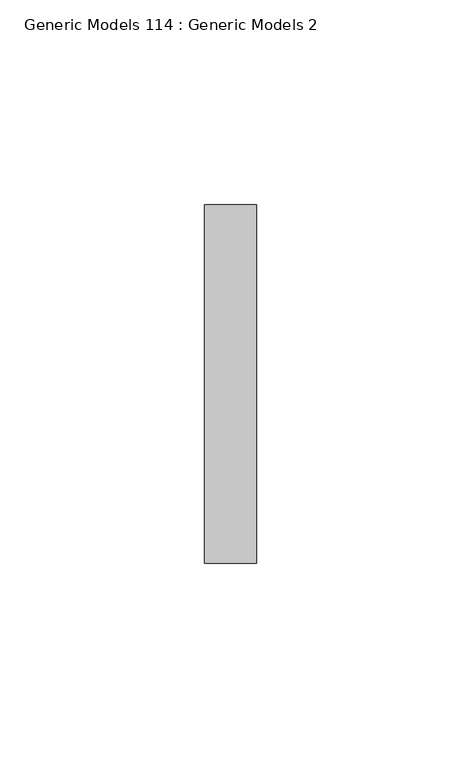
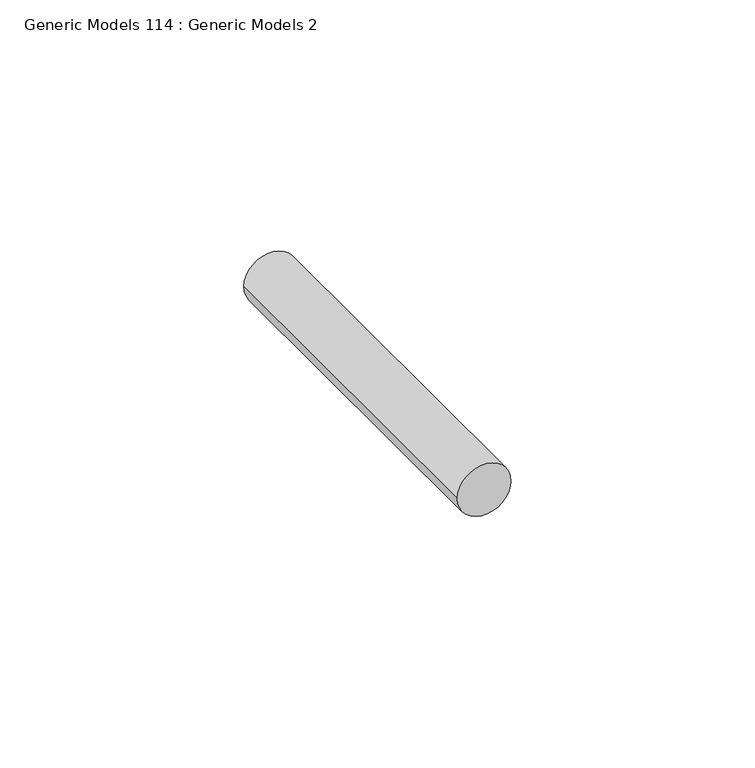
"""IFC4 building model written with IfcOpenShell, lengths in millimetres: proxy geometry, Generic Models 114 : Generic Models 2."""

from ifc_helpers import new_model, si_unit, point, frame, frame_2d, origin, place, context, project, spatial, circle_curve, trimmed, segment, composite_curve, outline, extrude, source, transform, mapped, element, save


def generic_models_114_generic_models_2_6e7f5802(model_context):
    return source(origin(), model_context, "Body", "SweptSolid", [
        extrude(outline(composite_curve([segment(trimmed(circle_curve(frame_2d((37860.4162436, 6848.7828124)), 6.35), [point((37860.4162436, 6842.4328124))], [point((37860.4162436, 6855.1328124))], False, "CARTESIAN"), True, "CONTINUOUS"), segment(trimmed(circle_curve(frame_2d((37860.4162436, 6848.7828124)), 6.35), [point((37860.4162436, 6855.1328124))], [point((37860.4162436, 6842.4328124))], False, "CARTESIAN"), True, "CONTINUOUS")], self_intersect=False)), frame((0.0, 1848.3666731, 0.0), z_axis=(0.0, 1.0, 0.0), x_axis=(0.0, 0.0, 1.0)), (0.0, 0.0, 1.0), 87.551022),
    ])


if __name__ == "__main__":
    model = new_model("IFC4")
    model_context = context("Model", 3, world=origin())
    ifc_project = project(units=[si_unit("LENGTHUNIT", "METRE", prefix="MILLI")], contexts=[model_context])
    site = spatial("IfcSite", under=ifc_project)
    building = spatial("IfcBuilding", under=site)
    placement = place(None, origin())
    generic_models_114_generic_models_2_shape = generic_models_114_generic_models_2_6e7f5802(model_context)
    element("IfcBuildingElementProxy", 1, Name="Generic Models 114 : Generic Models 2", ObjectType="Generic Models 114 : Generic Models 2", at=placement, inside=building, context=model_context, shape_type="MappedRepresentation", body=[
        mapped(generic_models_114_generic_models_2_shape, transform((0.0, 0.0, 0.0), x_axis=(1.0, 0.0, 0.0), y_axis=(0.0, 1.0, 0.0), z_axis=(0.0, 0.0, 1.0))),
    ])
    save(model, "model.ifc")

# Revit data of these elements
# Element 1 (IfcBuildingElementProxy, "Generic Models 114 : Generic Models 2")
#   Materials on its faces: "S.S. LAG BOLT - SEE STRUCT. DWGS"
# Materials
#   "S.S. LAG BOLT - SEE STRUCT. DWGS": class "Generic", colour RGB 120 120 120, transparency 0, Cost = 0
